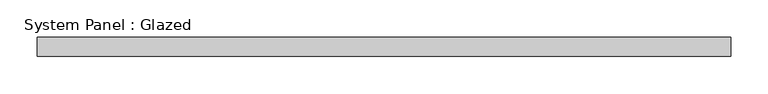
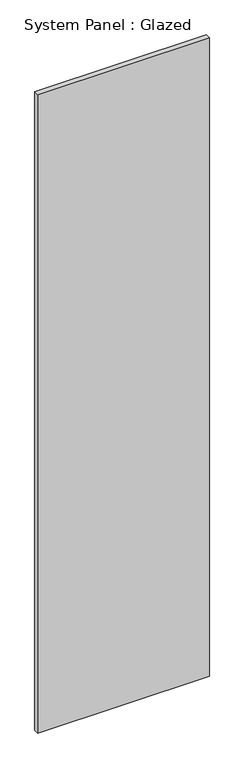
"""IFC4 building model written with IfcOpenShell, lengths in millimetres: plate geometry, System Panel : Glazed."""

import ifcopenshell
import ifcopenshell.guid

model = None  # the IFC model being written
_history = None  # IfcOwnerHistory: only IFC2X3 demands one
_inside = {}  # id of a spatial element -> (the spatial element, [elements in it])
_under = {}  # id of a project, library or spatial element -> (it, [spatial elements below it])
_declared = {}  # id of a project -> (the project, [libraries it declares])
_typed = {}  # id of a type object -> (the type object, [elements of that type])
_made_of = {}  # id of a material, layer set ... -> (it, [elements and type objects made of it])


def new_model(schema):
    """Start an empty IFC model of exactly this schema.

    Asked for "IFC4X3", IfcOpenShell would pick the latest addendum, in which some entities
    have other attributes; the version numbers below select the first issue.
    IFC2X3 requires an IfcOwnerHistory on every rooted entity: one is made here for all.
    """
    global model, _history
    if schema == "IFC4X3":
        model = ifcopenshell.file(schema_version=(4, 3, 0, 0))
    else:
        model = ifcopenshell.file(schema=schema)
    _inside.clear()
    _under.clear()
    _declared.clear()
    _typed.clear()
    _made_of.clear()
    _history = None
    if model.schema == "IFC2X3":
        org = make("IfcOrganization", Name="unknown")
        user = make(
            "IfcPersonAndOrganization",
            ThePerson=make("IfcPerson", FamilyName="unknown"),
            TheOrganization=org,
        )
        app = make(
            "IfcApplication",
            ApplicationDeveloper=org,
            Version="unknown",
            ApplicationFullName="unknown",
            ApplicationIdentifier="unknown",
        )
        _history = make(
            "IfcOwnerHistory",
            OwningUser=user,
            OwningApplication=app,
            ChangeAction="ADDED",
            CreationDate=0,
        )
    return model


def make(cls, **values):
    """One entity of the class cls with the attributes given. An attribute that is None is left unset."""
    return model.create_entity(
        cls, **{name: value for name, value in values.items() if value is not None}
    )


def rooted(cls, **values):
    """An entity with a GlobalId (a new one), such as an element, a storey or a relation."""
    return make(cls, GlobalId=ifcopenshell.guid.new(), OwnerHistory=_history, **values)


def si_unit(unit_type, name, prefix=None):
    """IfcSIUnit, for example si_unit("LENGTHUNIT", "METRE", prefix="MILLI")."""
    return make("IfcSIUnit", UnitType=unit_type, Prefix=prefix, Name=name)


def assignment(units):
    """IfcUnitAssignment: the units of a project."""
    return None if units is None else make("IfcUnitAssignment", Units=units)


def point(xyz):
    """IfcCartesianPoint."""
    return None if xyz is None else make("IfcCartesianPoint", Coordinates=xyz)


def direction(xyz):
    """IfcDirection."""
    return None if xyz is None else make("IfcDirection", DirectionRatios=xyz)


def frame(location, z_axis=None, x_axis=None):
    """IfcAxis2Placement3D, a coordinate frame: its origin and axes. An axis left out is left unset."""
    return make(
        "IfcAxis2Placement3D",
        Location=point(location),
        Axis=direction(z_axis),
        RefDirection=direction(x_axis),
    )


def origin():
    """The frame at (0, 0, 0) with its axes left unset."""
    return frame((0.0, 0.0, 0.0))


def origin_with_axes():
    """The frame at (0, 0, 0) with the z axis (0, 0, 1) and the x axis (1, 0, 0) written out."""
    return frame((0.0, 0.0, 0.0), z_axis=(0.0, 0.0, 1.0), x_axis=(1.0, 0.0, 0.0))


def place(relative_to, where):
    """IfcLocalPlacement: puts the frame where relative to a parent placement (None: the world)."""
    return make(
        "IfcLocalPlacement", PlacementRelTo=relative_to, RelativePlacement=where
    )


def context(
    kind, dimensions, precision=None, world=None, true_north=None, identifier=None
):
    """IfcGeometricRepresentationContext, for example the 3D "Model" context."""
    return make(
        "IfcGeometricRepresentationContext",
        ContextIdentifier=identifier,
        ContextType=kind,
        CoordinateSpaceDimension=dimensions,
        Precision=precision,
        WorldCoordinateSystem=world,
        TrueNorth=true_north,
    )


def project(units=None, contexts=None):
    """IfcProject with its units and contexts."""
    return rooted(
        "IfcProject",
        Name="project",
        RepresentationContexts=contexts,
        UnitsInContext=assignment(units),
    )


def spatial(cls, under=None, at=None, **own):
    """A site, building, storey or space (cls), placed at a placement, below another one or the project."""
    s = rooted(cls, ObjectPlacement=at, **own)
    if under is not None:
        _under.setdefault(under.id(), (under, []))[1].append(s)
    return s


def polyline(points):
    """IfcPolyline through the points."""
    return make("IfcPolyline", Points=[point(p) for p in points])


def outline(outer, holes=None, kind="AREA"):
    """IfcArbitraryClosedProfileDef: a profile drawn as a closed curve; with holes, ...WithVoids."""
    if holes is None:
        return make("IfcArbitraryClosedProfileDef", ProfileType=kind, OuterCurve=outer)
    return make(
        "IfcArbitraryProfileDefWithVoids",
        ProfileType=kind,
        OuterCurve=outer,
        InnerCurves=holes,
    )


def extrude(swept, where, along, depth):
    """IfcExtrudedAreaSolid: the profile swept, set in the frame where, extruded along a direction by depth."""
    return make(
        "IfcExtrudedAreaSolid",
        SweptArea=swept,
        Position=where,
        ExtrudedDirection=direction(along),
        Depth=depth,
    )


def shape(context_of_items, identifier, shape_type, items):
    """IfcShapeRepresentation: the items that make up one representation, for example the "Body"."""
    return make(
        "IfcShapeRepresentation",
        ContextOfItems=context_of_items,
        RepresentationIdentifier=identifier,
        RepresentationType=shape_type,
        Items=items,
    )


def source(mapping_origin, context_of_items, identifier, shape_type, items):
    """IfcRepresentationMap: a shape defined once, which mapped items show again and again."""
    return make(
        "IfcRepresentationMap",
        MappingOrigin=mapping_origin,
        MappedRepresentation=shape(context_of_items, identifier, shape_type, items),
    )


def transform(
    local_origin,
    x_axis=None,
    y_axis=None,
    z_axis=None,
    scale=None,
    scale2=None,
    scale3=None,
    uniform=True,
):
    """IfcCartesianTransformationOperator3D, or its non-uniform kind. x_axis, y_axis, z_axis: its Axis1, 2, 3."""
    if uniform:
        return make(
            "IfcCartesianTransformationOperator3D",
            Axis1=direction(x_axis),
            Axis2=direction(y_axis),
            LocalOrigin=point(local_origin),
            Scale=scale,
            Axis3=direction(z_axis),
        )
    return make(
        "IfcCartesianTransformationOperator3DnonUniform",
        Axis1=direction(x_axis),
        Axis2=direction(y_axis),
        LocalOrigin=point(local_origin),
        Scale=scale,
        Axis3=direction(z_axis),
        Scale2=scale2,
        Scale3=scale3,
    )


def mapped(mapping_source, mapping_target):
    """IfcMappedItem: shows the shape of a source again, moved by a transform."""
    return make(
        "IfcMappedItem", MappingSource=mapping_source, MappingTarget=mapping_target
    )


def made_of(thing, what):
    """Note that an element or type object is made of a material, layer set ...; save() writes the relation."""
    if what is not None:
        _made_of.setdefault(what.id(), (what, []))[1].append(thing)
    return thing


def element(
    cls,
    number,
    at=None,
    inside=None,
    cuts=None,
    type_object=None,
    material=None,
    context=None,
    identifier="Body",
    shape_type=None,
    held_by="IfcProductDefinitionShape",
    body=None,
    shapes=None,
    **own,
):
    """One element of the class cls, such as IfcWall. Its Tag is "e" and its number.

    at: its placement. inside: the storey or other place that contains it. cuts: it is an
    opening in that element (IfcRelVoidsElement). A single representation is given by context,
    identifier, shape_type and body (its items); several are given by shapes. held_by: the class
    of the entity that holds the representations. save() writes the other relations.
    """
    e = rooted(cls, Tag="e%d" % number, ObjectPlacement=at, **own)
    if body is not None:
        shapes = [shape(context, identifier, shape_type, body)]
    if shapes is not None:
        e.Representation = make(held_by, Representations=shapes)
    if inside is not None:
        _inside.setdefault(inside.id(), (inside, []))[1].append(e)
    if cuts is not None:
        rooted(
            "IfcRelVoidsElement", RelatingBuildingElement=cuts, RelatedOpeningElement=e
        )
    if type_object is not None:
        _typed.setdefault(type_object.id(), (type_object, []))[1].append(e)
    return made_of(e, material)


def aggregate(whole, parts):
    """IfcRelAggregates: a whole, such as a stair, and the parts it consists of."""
    return rooted("IfcRelAggregates", RelatingObject=whole, RelatedObjects=parts)


def save(model, path):
    """Write the relations noted so far, then the file.

    IfcRelAggregates (storeys below a building ...), IfcRelContainedInSpatialStructure (elements
    in a storey), IfcRelDefinesByType, IfcRelAssociatesMaterial and IfcRelDeclares: one each for
    every whole, place, type object, material and project.
    """
    for whole, parts in _under.values():
        aggregate(whole, parts)
    for where, things in _inside.values():
        rooted(
            "IfcRelContainedInSpatialStructure",
            RelatedElements=things,
            RelatingStructure=where,
        )
    for kind, things in _typed.values():
        rooted("IfcRelDefinesByType", RelatedObjects=things, RelatingType=kind)
    for what, things in _made_of.values():
        rooted("IfcRelAssociatesMaterial", RelatedObjects=things, RelatingMaterial=what)
    for by, libraries in _declared.values():
        rooted("IfcRelDeclares", RelatingContext=by, RelatedDefinitions=libraries)
    model.write(path)


def system_panel_glazed_b062bbc2(model_context):
    return source(origin(), model_context, "Body", "SweptSolid", [
        extrude(outline(polyline([(465.8483058, -44.45), (-465.8483058, -44.45), (-465.8483058, -19.05), (465.8483058, -19.05), (465.8483058, -44.45)])), origin_with_axes(), (0.0, 0.0, 1.0), 3657.6),
    ])


if __name__ == "__main__":
    model = new_model("IFC4")
    model_context = context("Model", 3, world=origin())
    ifc_project = project(units=[si_unit("LENGTHUNIT", "METRE", prefix="MILLI")], contexts=[model_context])
    site = spatial("IfcSite", under=ifc_project)
    building = spatial("IfcBuilding", under=site)
    placement = place(None, origin())
    system_panel_glazed_shape = system_panel_glazed_b062bbc2(model_context)
    element("IfcPlate", 1, ObjectType="System Panel : Glazed", at=placement, inside=building, context=model_context, shape_type="MappedRepresentation", body=[
        mapped(system_panel_glazed_shape, transform((0.0, 0.0, 0.0), x_axis=(1.0, 0.0, 0.0), y_axis=(0.0, 1.0, 0.0), z_axis=(0.0, 0.0, 1.0))),
    ])
    save(model, "model.ifc")

# Revit data of these elements
# Type "System Panel : Glazed"
#   Construction Type Id = "GSP4R"
#   Analytic Construction = "1/8 in Pilkington single glazing"
#   Visual Light Transmittance = 0.9
#   Solar Heat Gain Coefficient = 0.86
#   Heat Transfer Coefficient (U) = 1.18115 BTU/(h·ft²·°F)
#   Define Thermal Properties by = 1
# Element 1 (IfcPlate, "System Panel : Glazed")
#   Materials on its faces: "Glass"
# Materials
#   "Glass": class "Glass", colour RGB 0 128 192, transparency 0.75, Description = "Soda Lime Glass", Cost = 0
